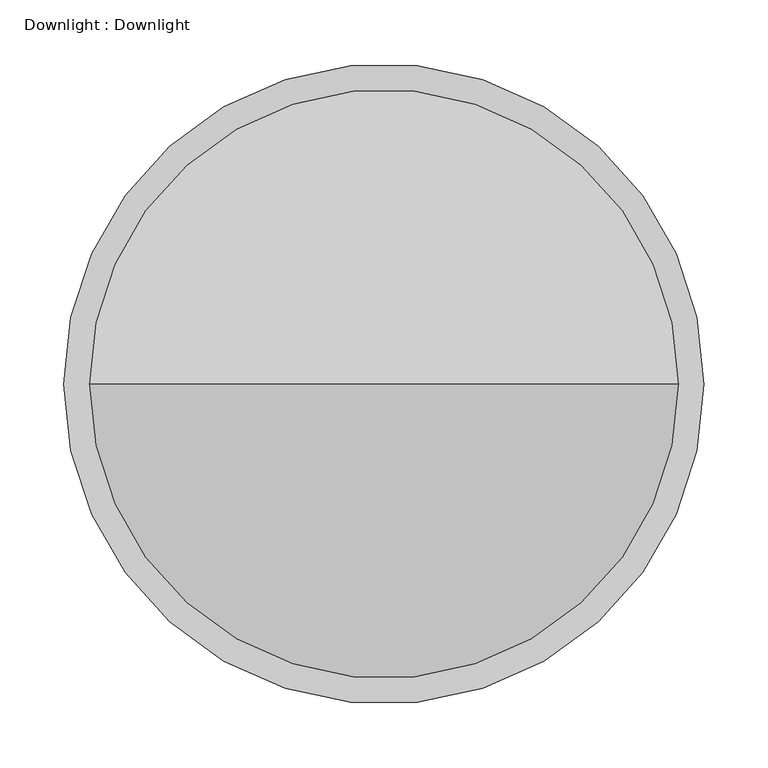
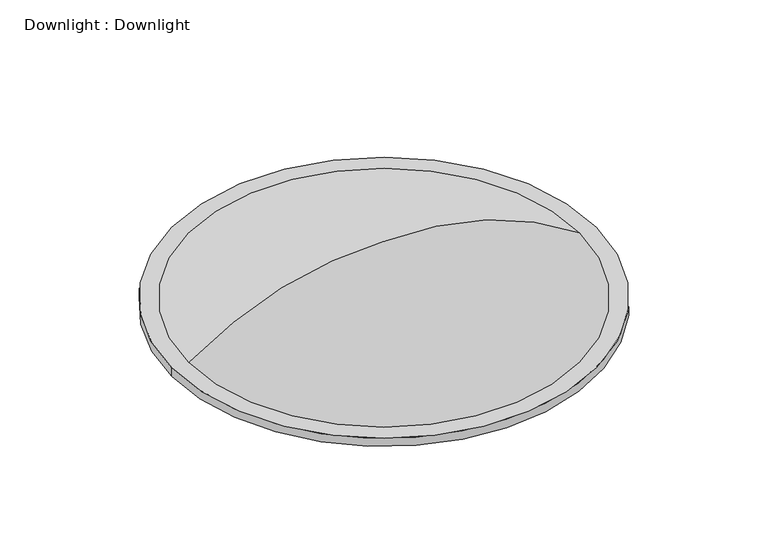
"""IFC4 building model written with IfcOpenShell, lengths in millimetres: light fixture geometry, Downlight : Downlight."""

from ifc_helpers import new_model, si_unit, point, frame, origin, origin_2d, place, context, project, spatial, circle_curve, ellipse_curve, trimmed, segment, composite_curve, outline, extrude, source, transform, mapped, element, save
from ifc_brep_helpers import plane_surface, revolved_surface, advanced_brep


def downlight_downlight_e6a68a7d(model_context):
    return source(origin(), model_context, "Body", "SolidModel", [
        advanced_brep(
        [(-230.0, 0.0, 0.0), (230.0, 0.0, 0.0), (0.0, 0.0, 0.0), (0.0, 0.0, 70.3180567)],
        [
            (0, 1, circle_curve(frame((0.0, 0.0, 0.0), z_axis=(0.0, 0.0, -1.0), x_axis=(1.0, 0.0, 0.0)), 230.0)),
            (1, 2),
            (2, 0),
            (1, 0, circle_curve(frame((0.0, 0.0, 0.0), z_axis=(0.0, 0.0, -1.0), x_axis=(1.0, 0.0, 0.0)), 230.0)),
            (3, 1, circle_curve(frame((13.1969865, 0.0, -297.8236248), z_axis=(0.0, 1.0, 0.0), x_axis=(1.0, 0.0, 0.0)), 368.3781456)),
            (0, 3, circle_curve(frame((-13.1969865, 0.0, -297.8236248), z_axis=(0.0, 1.0, 0.0), x_axis=(-1.0, 0.0, 0.0)), 368.3781456)),
        ],
        [
            plane_surface(frame((0.0, 0.0, 0.0), z_axis=(0.0, 0.0, -1.0), x_axis=(1.0, 0.0, 0.0))),
            revolved_surface(trimmed(ellipse_curve(frame((13.1969865, 0.0, -297.8236248), z_axis=(0.0, -1.0, 0.0), x_axis=(1.0, 0.0, 0.0)), 368.3781456, 368.3781456), [point((230.0, 0.0, 0.0))], [point((0.0, 0.0, 70.3180567))], True, "CARTESIAN"), (0.0, 0.0, 2194.0651339), (0.0, 0.0, 1.0)),
        ],
        [
            (0, [[1, 2, 3]]),
            (0, [[4, -3, -2]]),
            (1, [[5, -1, 6]]),
            (1, [[-6, -4, -5]]),
        ],
    ),
        extrude(outline(composite_curve([segment(trimmed(circle_curve(origin_2d(), 250.0), [point((-250.0, 0.0))], [point((250.0, 0.0))], False, "CARTESIAN"), True, "CONTINUOUS"), segment(trimmed(circle_curve(origin_2d(), 250.0), [point((250.0, 0.0))], [point((-250.0, 0.0))], False, "CARTESIAN"), True, "CONTINUOUS")], self_intersect=False)), frame((0.0, 0.0, -10.1537533), z_axis=(0.0, 0.0, 1.0), x_axis=(1.0, 0.0, 0.0)), (0.0, 0.0, 1.0), 10.1537533),
    ])


if __name__ == "__main__":
    model = new_model("IFC4")
    model_context = context("Model", 3, world=origin())
    ifc_project = project(units=[si_unit("LENGTHUNIT", "METRE", prefix="MILLI")], contexts=[model_context])
    site = spatial("IfcSite", under=ifc_project)
    building = spatial("IfcBuilding", under=site)
    placement = place(None, origin())
    downlight_downlight_shape = downlight_downlight_e6a68a7d(model_context)
    element("IfcLightFixture", 1, ObjectType="Downlight : Downlight", at=placement, inside=building, context=model_context, shape_type="MappedRepresentation", body=[
        mapped(downlight_downlight_shape, transform((0.0, 0.0, 0.0), x_axis=(1.0, 0.0, 0.0), y_axis=(0.0, 1.0, 0.0), z_axis=(0.0, 0.0, 1.0))),
    ])
    save(model, "model.ifc")

# Revit data of these elements
# Type "Downlight : Downlight"
#   Default Elevation = 0
